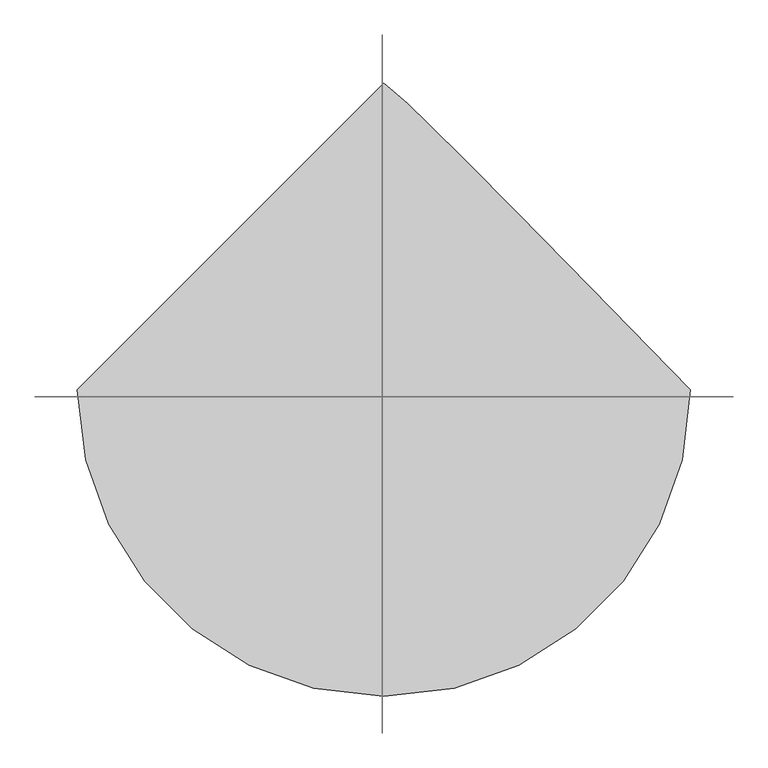
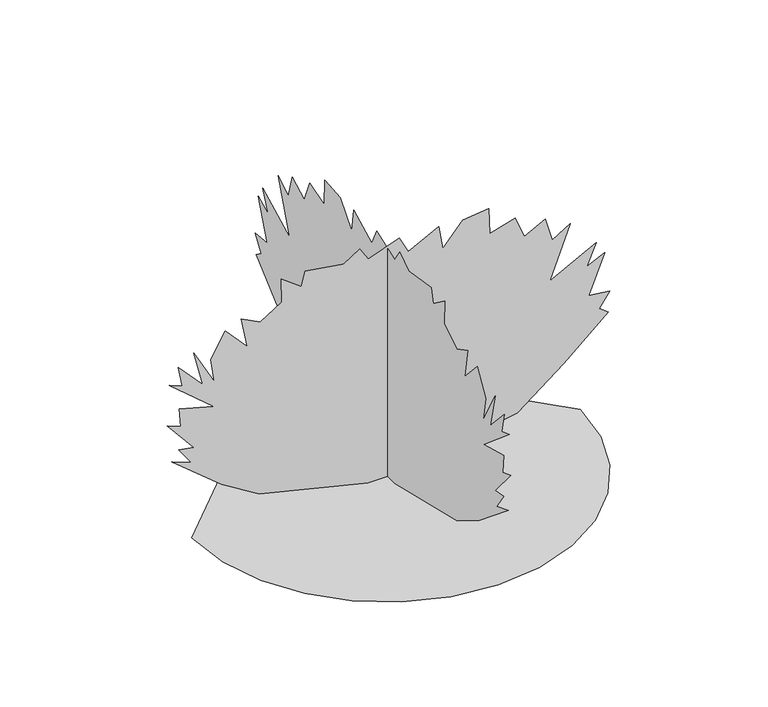
"""IFC4 building model written with IfcOpenShell, lengths in millimetres: proxy geometry, yew 26768 : yew 26768."""

from ifc_helpers import new_model, si_unit, origin, place, context, project, spatial, triangles, source, transform, mapped, element, save


def entourage_1708232a(model_context):
    return source(origin(), model_context, "Body", "Tessellation", [
        triangles([(-552.1733454, 0.0, 5.4e-06), (-537.5734008, -126.5215106, 5.4e-06), (-496.001229, -242.7110573, 5.4e-06), (-430.7790836, -345.2394648, 5.4e-06), (-345.2394648, -430.7790836, 5.4e-06), (-242.7110573, -496.001229, 5.4e-06), (-126.5212562, -537.5734008, 5.4e-06), (2.41e-05, -552.1733454, 5.4e-06), (126.5215106, -537.5734008, 5.4e-06), (242.7110573, -496.001229, 5.4e-06), (345.2394648, -430.7790836, 5.4e-06), (430.7790836, -345.2394648, 5.4e-06), (496.001229, -242.7110573, 5.4e-06), (537.5734008, -126.5212562, 5.4e-06), (552.1733454, 4.83e-05, 5.4e-06), (372.7273582, 184.0654909, 5.4e-06), (239.6978509, 319.5854711, 5.4e-06), (145.3449528, 414.6475465, 5.4e-06), (81.9343338, 477.3474621, 5.4e-06), (41.7301836, 515.775131, 5.4e-06), (16.9973058, 538.0179231, 5.4e-06), (-7.24e-05, 552.1733454, 5.4e-06), (-57.9623142, -12.396627, 5.21e-05), (-367.0047423, -12.396652, 75.5734076), (-474.5509031, -12.396652, 142.0056127), (-616.6665018, -12.396652, 259.1080397), (-561.3351408, -12.396652, 237.5164979), (-596.4227157, -12.396652, 287.4493694), (-553.2375973, -12.396652, 279.351844), (-628.8127808, -12.396652, 371.1195348), (-591.025189, -12.396652, 356.2757824), (-595.0739608, -12.396652, 410.2558814), (-496.5574814, -12.396652, 383.2658137), (-623.412747, -12.3966781, 491.2285552), (-585.6276987, -12.3966781, 476.3822594), (-597.7714342, -12.3966781, 535.7623921), (-527.5962845, -12.3966781, 460.1872087), (-553.2375973, -12.3966781, 564.1011784), (-495.2087265, -12.3966781, 457.4897352), (-506.0037435, -12.3966781, 527.6648849), (-464.1699234, -12.3966781, 599.1887532), (-402.0923172, -12.3966781, 530.3649018), (-418.2848245, -12.3966781, 619.4325394), (-364.3047255, -12.3966781, 591.091246), (-303.5758378, -12.3966781, 630.2275927), (-304.9245564, -12.3966781, 699.0539875), (-248.2454578, -12.3966781, 657.2201311), (-237.4491873, -12.3966781, 699.0539875), (-126.787955, -12.3966781, 681.5102182), (-82.2536094, -12.3966781, 711.2002665), (-57.9623142, -12.3966781, 673.4126747), (29.7568728, -12.3966781, 705.8027761), (55.3245209, -12.3966781, 655.0738958), (143.2032231, -12.3966781, 700.044552), (153.8874819, -12.3966781, 630.387612), (210.5935046, -12.3966781, 696.3564777), (284.8179166, -12.3966781, 704.4514778), (287.5154082, -12.3966781, 628.8788378), (360.3905748, -12.3966781, 649.1226603), (386.0318876, -12.3966781, 584.3450008), (445.4120204, -12.3966781, 616.7325588), (465.6532994, -12.3966781, 546.5574091), (515.5871701, -12.3966781, 578.9474742), (457.5557559, -12.396652, 426.4509321), (589.8110916, -12.3966781, 495.2747835), (562.8184805, -12.396652, 433.197141), (614.1011061, -12.3966781, 457.4897352), (568.2185143, -12.396652, 344.1295034), (628.9474382, -12.396652, 336.0319599), (597.9085988, -12.396652, 294.1956146), (623.5474045, -12.396652, 275.3030723), (498.0433645, -12.396652, 164.6420943), (365.7880651, -12.396652, 62.0781285), (289.9233281, -12.396652, 47.6486405), (164.5613216, -12.396652, 15.2766327), (36.5046395, -12.396627, 1.4e-05), (-3.3569921, -47.7068037, 4.09e-05), (-3.3569921, -356.74821, 75.5734076), (-3.3569921, -464.2969142, 142.0056127), (-3.3569921, -606.4099694, 259.1080397), (-3.3569921, -551.0786084, 237.5164979), (-3.3569921, -586.1687267, 287.4493694), (-3.3569921, -542.9836083, 279.351844), (-3.3569921, -618.5562847, 371.1195348), (-3.3569921, -580.7686566, 356.2757824), (-3.3569921, -584.8174284, 410.2558814), (-3.3569921, -486.3034925, 383.2658137), (-3.3569921, -613.1587944, 491.2285552), (-3.3569921, -575.3711663, 476.3822594), (-3.3569669, -587.5174453, 535.7623921), (-3.3569921, -517.3422956, 460.1872087), (-3.3569669, -542.9836083, 564.1011784), (-3.3569921, -484.9522305, 457.4897352), (-3.3569921, -495.7497545, 527.6648849), (-3.3569669, -453.913391, 599.1887532), (-3.3569921, -391.8357848, 530.3649018), (-3.3569669, -408.0308355, 619.4325394), (-3.3569921, -354.0481931, 591.091246), (-3.3569921, -293.3193054, 630.2275927), (-3.3569669, -294.6705856, 699.0539875), (-3.3569921, -237.9897067, 657.2201311), (-3.3569669, -227.1936905, 699.0539875), (-3.3569921, -116.5324491, 681.5102182), (-3.3569921, -71.9981035, 711.2002665), (-3.3569921, -47.7068037, 673.4126747), (-3.3569921, 40.0126331, 705.8027761), (-3.3569921, 65.5800314, 655.0738958), (-3.3569921, 153.458729, 700.044552), (-3.3569921, 164.1429969, 630.387612), (-3.3569921, 220.8490196, 696.3564777), (-3.3569921, 295.0719056, 704.4514778), (-3.3569921, 297.7719224, 628.8788378), (-3.3569921, 370.6471072, 649.1226603), (-3.3569921, 396.28842, 584.3450008), (-3.3569921, 455.6660093, 616.7325588), (-3.3569921, 475.9098318, 546.5574091), (-3.3569921, 525.8411591, 578.9474742), (-3.3569921, 467.8122883, 426.4509321), (-3.3569921, 600.0650442, 495.2747835), (-3.3569921, 573.0750129, 433.197141), (-3.3569921, 624.3576021, 457.4897352), (-3.3569921, 578.4725032, 344.1295034), (-3.3569921, 639.2013908, 336.0319599), (-3.3569921, 608.1625877, 294.1956146), (-3.3569921, 633.8039005, 275.3030723), (-3.3570177, 508.2973535, 164.6420943), (-3.3570177, 376.0445975, 62.0781285), (-3.3570177, 300.1798423, 47.6486405), (-3.3569921, 174.8168366, 15.2766327), (-3.3569921, 46.7601454, 0.0)], [[21, 22, 1], [20, 21, 1], [19, 20, 1], [18, 19, 1], [17, 18, 1], [17, 1, 2], [17, 2, 3], [17, 3, 4], [16, 17, 4], [16, 4, 5], [16, 5, 6], [16, 6, 7], [16, 7, 8], [16, 8, 9], [16, 9, 10], [16, 10, 11], [16, 11, 12], [15, 16, 12], [14, 15, 12], [13, 14, 12], [37, 38, 39], [25, 26, 27], [33, 34, 35], [29, 30, 31], [35, 36, 37], [33, 35, 37], [62, 63, 64], [64, 65, 66], [66, 67, 68], [27, 28, 29], [42, 43, 44], [45, 46, 47], [68, 69, 70], [33, 37, 39], [31, 32, 33], [53, 54, 55], [40, 41, 42], [60, 61, 62], [70, 71, 72], [29, 31, 33], [39, 40, 42], [56, 57, 58], [49, 50, 51], [55, 56, 58], [64, 66, 68], [47, 48, 49], [58, 59, 60], [51, 52, 53], [60, 62, 64], [68, 70, 72], [64, 68, 72], [64, 72, 73], [64, 73, 74], [25, 27, 29], [25, 29, 33], [24, 25, 33], [23, 24, 33], [64, 74, 75], [60, 64, 75], [58, 60, 75], [55, 58, 75], [55, 75, 76], [53, 55, 76], [53, 76, 23], [53, 23, 33], [51, 53, 33], [49, 51, 33], [47, 49, 33], [45, 47, 33], [33, 39, 42], [45, 33, 42], [44, 45, 42], [91, 92, 93], [79, 80, 81], [87, 88, 89], [83, 84, 85], [89, 90, 91], [87, 89, 91], [116, 117, 118], [118, 119, 120], [120, 121, 122], [81, 82, 83], [96, 97, 98], [99, 100, 101], [122, 123, 124], [87, 91, 93], [85, 86, 87], [107, 108, 109], [94, 95, 96], [114, 115, 116], [124, 125, 126], [83, 85, 87], [93, 94, 96], [110, 111, 112], [103, 104, 105], [109, 110, 112], [118, 120, 122], [101, 102, 103], [112, 113, 114], [105, 106, 107], [114, 116, 118], [122, 124, 126], [118, 122, 126], [118, 126, 127], [118, 127, 128], [79, 81, 83], [79, 83, 87], [78, 79, 87], [77, 78, 87], [118, 128, 129], [114, 118, 129], [112, 114, 129], [109, 112, 129], [109, 129, 130], [107, 109, 130], [107, 130, 77], [107, 77, 87], [105, 107, 87], [103, 105, 87], [101, 103, 87], [99, 101, 87], [87, 93, 96], [99, 87, 96], [98, 99, 96]], closed=False),
    ])


if __name__ == "__main__":
    model = new_model("IFC4")
    model_context = context("Model", 3, world=origin())
    ifc_project = project(units=[si_unit("LENGTHUNIT", "METRE", prefix="MILLI")], contexts=[model_context])
    site = spatial("IfcSite", under=ifc_project)
    building = spatial("IfcBuilding", under=site)
    placement = place(None, origin())
    entourage_shape = entourage_1708232a(model_context)
    element("IfcBuildingElementProxy", 1, Name="yew 26768 : yew 26768", ObjectType="yew 26768 : yew 26768", at=placement, inside=building, context=model_context, shape_type="MappedRepresentation", body=[
        mapped(entourage_shape, transform((0.0, 0.0, 0.0), x_axis=(1.0, 0.0, 0.0), y_axis=(0.0, 1.0, 0.0), z_axis=(0.0, 0.0, 1.0))),
    ])
    save(model, "model.ifc")

# Revit data of these elements
# Type "yew 26768 : yew 26768"
#   built-in parameter 1005195 = "RPC-16-FWJ8-ELQ0-EHM0-2000-ST1L-LVER-AU"
#   Height = 0
